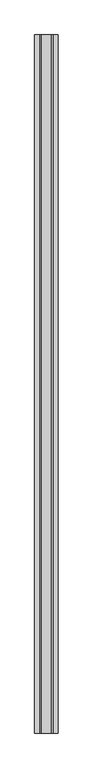
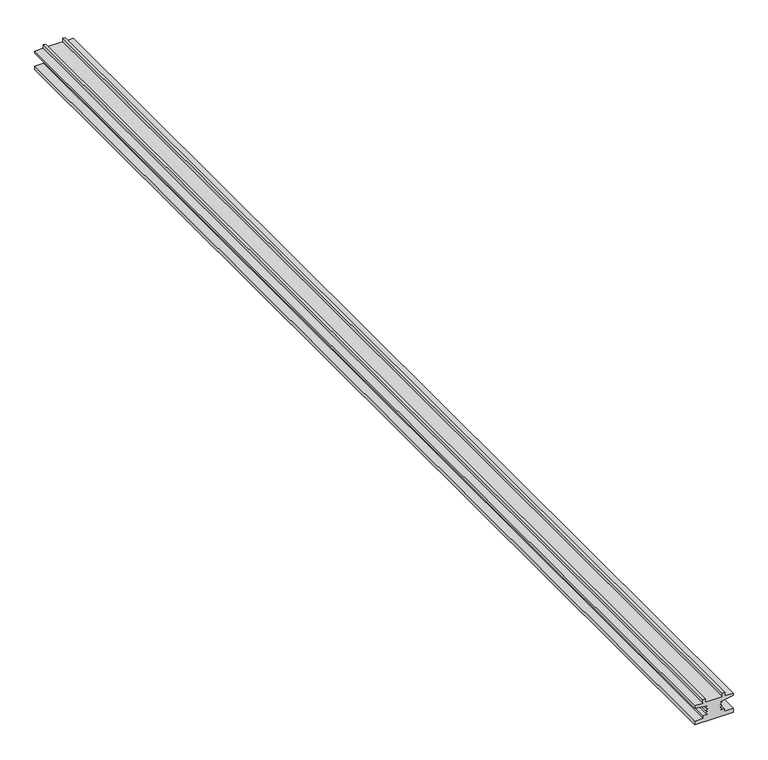
"""IFC4 building model written with IfcOpenShell, lengths in millimetres: proxy geometry, Bison pedestal005 : Bison pedestal005."""

from ifc_helpers import new_model, si_unit, frame, origin, place, context, project, spatial, polyline, outline, extrude, source, transform, mapped, element, save


def generic_models_73726d1c(model_context):
    return source(origin(), model_context, "Body", "SweptSolid", [
        extrude(outline(polyline([(36480.0342739, -2164.2674432), (36486.734375, -2164.2028809), (36486.734375, -2179.6223145), (36491.2120625, -2179.6223145), (36491.2120625, -2187.7133789), (36494.1534688, -2184.1826172), (36496.7296406, -2187.4926758), (36499.4503438, -2183.9621582), (36502.0245625, -2187.3457031), (36504.5577656, -2183.7709961), (36507.1046406, -2186.9875488), (36510.9913594, -2164.2028809), (36515.1456563, -2164.2028809), (36515.1456563, -2178.9460449), (36521.3116719, -2178.9460449), (36521.3116719, -2182.8327637), (36515.1456563, -2182.8327637), (36515.1456563, -2213.1228027), (36521.3116719, -2213.1228027), (36521.3116719, -2217.0095215), (36515.1456563, -2217.0095215), (36515.1456563, -2231.7526855), (36510.9913594, -2231.7526855), (36507.1046406, -2208.9680176), (36504.5577656, -2212.1845703), (36502.0245625, -2208.6098633), (36499.4503438, -2211.9934082), (36496.7296406, -2208.4628906), (36494.1534688, -2211.7729492), (36491.2120625, -2208.2421875), (36491.2120625, -2216.333252), (36486.734375, -2216.333252), (36486.734375, -2231.7526855), (36480.0342739, -2231.6881232), (36480.0342739, -2164.2674432)])), frame((0.0, 998.1570053, 0.0), z_axis=(0.0, 1.0, 0.0), x_axis=(0.0, 0.0, 1.0)), (0.0, 0.0, 1.0), 2000.0),
    ])


if __name__ == "__main__":
    model = new_model("IFC4")
    model_context = context("Model", 3, world=origin())
    ifc_project = project(units=[si_unit("LENGTHUNIT", "METRE", prefix="MILLI")], contexts=[model_context])
    site = spatial("IfcSite", under=ifc_project)
    building = spatial("IfcBuilding", under=site)
    placement = place(None, origin())
    generic_models_shape = generic_models_73726d1c(model_context)
    element("IfcBuildingElementProxy", 1, Name="Bison pedestal005 : Bison pedestal005", ObjectType="Bison pedestal005 : Bison pedestal005", at=placement, inside=building, context=model_context, shape_type="MappedRepresentation", body=[
        mapped(generic_models_shape, transform((0.0, 0.0, 0.0), x_axis=(1.0, 0.0, 0.0), y_axis=(0.0, 1.0, 0.0), z_axis=(0.0, 0.0, 1.0))),
    ])
    save(model, "model.ifc")

# Revit data of these elements
# Type "Bison pedestal005 : Bison pedestal005"
#   NameOverride = "Bison pedestal005"
# Element 1 (IfcBuildingElementProxy, "Bison pedestal005 : Bison pedestal005")
#   Materials on its faces: "BUZON PEDESTAL"
# Materials
#   "BUZON PEDESTAL": class "Unassigned", colour RGB 66 66 66, transparency 0
